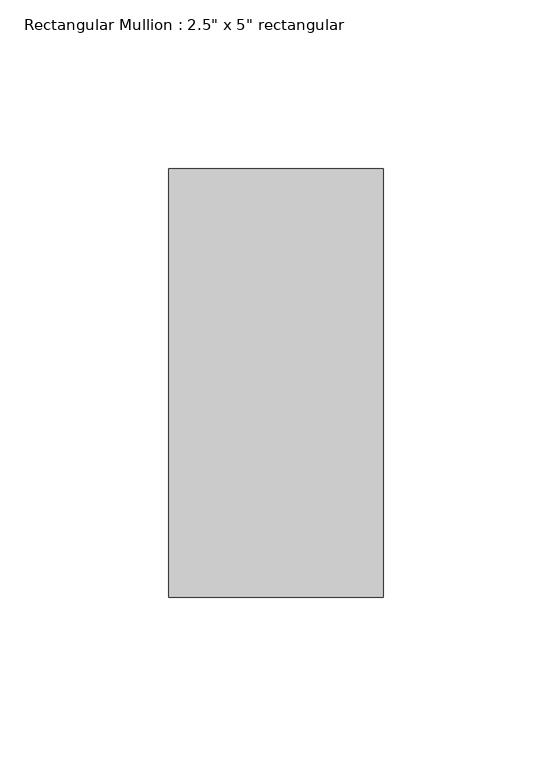
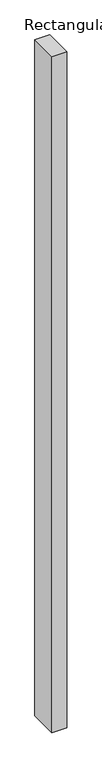
"""IFC4 building model written with IfcOpenShell, lengths in millimetres: member geometry."""

from ifc_helpers import new_model, si_unit, frame, origin, place, context, project, spatial, polyline, outline, extrude, source, transform, mapped, element, save


def member_6fa634db(model_context):
    return source(origin(), model_context, "Body", "SweptSolid", [
        extrude(outline(polyline([(31.75, 63.5), (31.75, -63.5), (-31.75, -63.5), (-31.75, 63.5), (31.75, 63.5)])), frame((0.0, 0.0, -3086.1), z_axis=(0.0, 0.0, 1.0), x_axis=(1.0, 0.0, 0.0)), (0.0, 0.0, 1.0), 3086.1),
    ])


if __name__ == "__main__":
    model = new_model("IFC4")
    model_context = context("Model", 3, world=origin())
    ifc_project = project(units=[si_unit("LENGTHUNIT", "METRE", prefix="MILLI")], contexts=[model_context])
    site = spatial("IfcSite", under=ifc_project)
    building = spatial("IfcBuilding", under=site)
    placement = place(None, origin())
    member_shape = member_6fa634db(model_context)
    element("IfcMember", 1, ObjectType="Rectangular Mullion : 2.5\" x 5\" rectangular", at=placement, inside=building, context=model_context, shape_type="MappedRepresentation", body=[
        mapped(member_shape, transform((0.0, 0.0, 0.0), x_axis=(1.0, 0.0, 0.0), y_axis=(0.0, 1.0, 0.0), z_axis=(0.0, 0.0, 1.0))),
    ])
    save(model, "model.ifc")

# Revit data of these elements
# Type "Rectangular Mullion : 2.5\" x 5\" rectangular"
#   built-in parameter 1007304 = 0.416667 (stored number, unit not read)
#   built-in parameter 1007301 = 0.104167 (stored number, unit not read)
#   built-in parameter 1007300 = 0.104167 (stored number, unit not read)
# Element 1 (IfcMember, "Rectangular Mullion : 2.5\" x 5\" rectangular")
#   Materials on its faces: "Aluminum"
# Materials
#   "Aluminum": class "Metal", colour RGB 247 247 247, transparency 0, Description = "Aluminum 6061", Cost = 0
